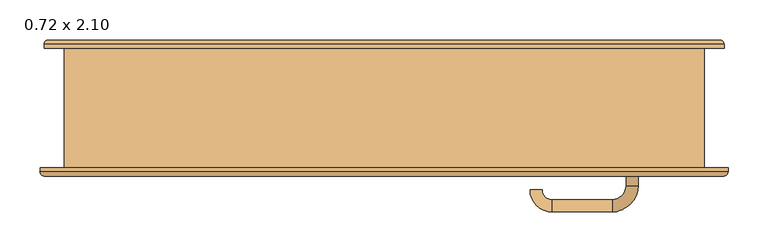
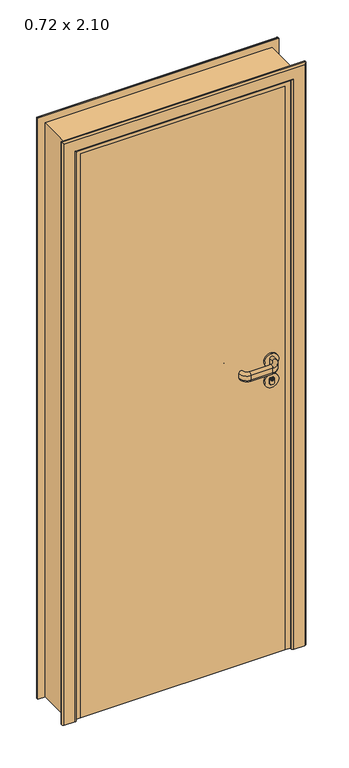
"""IFC4 building model written with IfcOpenShell, lengths in millimetres: door geometry, CC_PORTA ABRIR_1 FOLHA LISA : 0.72 x 2.10."""

from ifc_helpers import new_model, si_unit, point, frame, frame_2d, origin, origin_with_axes, place, context, project, spatial, polyline, circle_curve, ellipse_curve, trimmed, segment, composite_curve, outline, extrude, faceted_brep, source, transform, mapped, element, save
from ifc_brep_helpers import plane_surface, cylinder_surface, revolved_surface, advanced_brep


def door_0_72_x_2_10_8ac540cf(model_context):
    return source(origin(), model_context, "Body", "SolidModel", [
        advanced_brep(
        [(302.5, -40.0, 1091.5062746), (317.5, -40.0, 1091.5062746), (317.5, -40.0, 1108.3826844), (302.5, -40.0, 1108.3826844), (317.5, -18.0, 1091.5062746), (317.5, -18.0, 1108.3826844), (302.5, -18.0, 1108.3826844), (302.5, -18.0, 1091.5062746), (285.0, 14.5, 1108.3826844), (285.0, 14.5, 1091.5062746), (210.0, 14.5, 1091.5062746), (210.0, 14.5, 1108.3826844), (285.0, -0.5, 1091.5062746), (285.0, -0.5, 1108.3826844), (210.0, -0.5, 1108.3826844), (210.0, -0.5, 1091.5062746), (197.5, -13.0, 1091.5062746), (197.5, -13.0, 1108.3826844), (182.5, -13.0, 1108.3826844), (182.5, -13.0, 1091.5062746)],
        [
            (0, 1, circle_curve(frame((310.0, -40.0, 1091.5062746), z_axis=(0.0, -1.0, 0.0), x_axis=(0.0, 0.0, 1.0)), 7.5)),
            (1, 2),
            (2, 3, circle_curve(frame((310.0, -40.0, 1108.3826844), z_axis=(0.0, -1.0, 0.0), x_axis=(0.0, 0.0, 1.0)), 7.5)),
            (3, 0),
            (1, 4),
            (4, 5),
            (5, 2),
            (3, 6),
            (6, 7),
            (7, 0),
            (8, 9),
            (9, 10),
            (10, 11),
            (11, 8),
            (12, 13),
            (13, 14),
            (14, 15),
            (15, 12),
            (7, 4, circle_curve(frame((310.0, -18.0, 1091.5062746), z_axis=(0.0, -1.0, 0.0), x_axis=(0.0, 0.0, 1.0)), 7.5)),
            (5, 6, circle_curve(frame((310.0, -18.0, 1108.3826844), z_axis=(0.0, -1.0, 0.0), x_axis=(0.0, 0.0, 1.0)), 7.5)),
            (9, 12, circle_curve(frame((285.0, 7.0, 1091.5062746), z_axis=(-1.0, 0.0, 0.0), x_axis=(0.0, 0.0, 1.0)), 7.5)),
            (15, 10, circle_curve(frame((210.0, 7.0, 1091.5062746), z_axis=(1.0, 0.0, 0.0), x_axis=(0.0, 0.0, 1.0)), 7.5)),
            (13, 8, circle_curve(frame((285.0, 7.0, 1108.3826844), z_axis=(-1.0, 0.0, 0.0), x_axis=(0.0, 0.0, 1.0)), 7.5)),
            (11, 14, circle_curve(frame((210.0, 7.0, 1108.3826844), z_axis=(1.0, 0.0, 0.0), x_axis=(0.0, 0.0, 1.0)), 7.5)),
            (9, 4, circle_curve(frame((285.0, -18.0, 1091.5062746), z_axis=(0.0, 0.0, -1.0), x_axis=(1.0, 0.0, 0.0)), 32.5)),
            (7, 12, circle_curve(frame((285.0, -18.0, 1091.5062746), z_axis=(0.0, 0.0, 1.0), x_axis=(1.0, 0.0, 0.0)), 17.5)),
            (8, 5, circle_curve(frame((285.0, -18.0, 1108.3826844), z_axis=(0.0, 0.0, -1.0), x_axis=(1.0, 0.0, 0.0)), 32.5)),
            (13, 6, circle_curve(frame((285.0, -18.0, 1108.3826844), z_axis=(0.0, 0.0, -1.0), x_axis=(1.0, 0.0, 0.0)), 17.5)),
            (16, 17),
            (17, 18, circle_curve(frame((190.0, -13.0, 1108.3826844), z_axis=(0.0, -1.0, 0.0), x_axis=(0.0, 0.0, 1.0)), 7.5)),
            (18, 19),
            (19, 16, circle_curve(frame((190.0, -13.0, 1091.5062746), z_axis=(0.0, -1.0, 0.0), x_axis=(0.0, 0.0, 1.0)), 7.5)),
            (19, 10, circle_curve(frame((210.0, -13.0, 1091.5062746), z_axis=(0.0, 0.0, -1.0), x_axis=(0.0, 1.0, 0.0)), 27.5)),
            (15, 16, circle_curve(frame((210.0, -13.0, 1091.5062746), z_axis=(0.0, 0.0, 1.0), x_axis=(0.0, 1.0, 0.0)), 12.5)),
            (18, 11, circle_curve(frame((210.0, -13.0, 1108.3826844), z_axis=(0.0, 0.0, -1.0), x_axis=(0.0, 1.0, 0.0)), 27.5)),
            (17, 14, circle_curve(frame((210.0, -13.0, 1108.3826844), z_axis=(0.0, 0.0, -1.0), x_axis=(0.0, 1.0, 0.0)), 12.5)),
        ],
        [
            plane_surface(frame((310.0, -40.0, 1099.9444795), z_axis=(0.0, -1.0, 0.0), x_axis=(0.0, 0.0, 1.0))),
            plane_surface(frame((317.5, -40.0, 1091.5062746), z_axis=(1.0, 0.0, 0.0), x_axis=(0.0, 1.0, 0.0))),
            plane_surface(frame((302.5, -40.0, 1108.3826844), z_axis=(-1.0, 0.0, 0.0), x_axis=(0.0, 1.0, 0.0))),
            plane_surface(frame((285.0, 14.5, 1091.5062746), z_axis=(0.0, 1.0, 0.0), x_axis=(-1.0, 0.0, 0.0))),
            plane_surface(frame((285.0, -0.5, 1108.3826844), z_axis=(0.0, -1.0, 0.0), x_axis=(-1.0, 0.0, 0.0))),
            cylinder_surface(frame((310.0, -40.0, 1091.5062746), z_axis=(0.0, -1.0, 0.0), x_axis=(0.0, 0.0, 1.0)), 7.5),
            cylinder_surface(frame((310.0, -40.0, 1108.3826844), z_axis=(0.0, -1.0, 0.0), x_axis=(0.0, 0.0, 1.0)), 7.5),
            cylinder_surface(frame((285.0, 7.0, 1091.5062746), z_axis=(1.0, 0.0, 0.0), x_axis=(0.0, 0.0, 1.0)), 7.5),
            cylinder_surface(frame((285.0, 7.0, 1108.3826844), z_axis=(1.0, 0.0, 0.0), x_axis=(0.0, 0.0, 1.0)), 7.5),
            revolved_surface(trimmed(ellipse_curve(frame((310.0, -18.0, 1091.5062746), z_axis=(0.0, -1.0, 0.0), x_axis=(0.0, 0.0, 1.0)), 7.5, 7.5), [point((302.5, -18.0, 1091.5062746))], [point((317.5, -18.0, 1091.5062746))], True, "CARTESIAN"), (285.0, -18.0, 1099.9444795), (0.0, 0.0, 1.0)),
            cylinder_surface(frame((285.0, -18.0, 1099.9444795), z_axis=(0.0, 0.0, 1.0), x_axis=(1.0, 0.0, 0.0)), 32.5),
            revolved_surface(trimmed(ellipse_curve(frame((310.0, -18.0, 1108.3826844), z_axis=(0.0, -1.0, 0.0), x_axis=(0.0, 0.0, 1.0)), 7.5, 7.5), [point((317.5, -18.0, 1108.3826844))], [point((302.5, -18.0, 1108.3826844))], True, "CARTESIAN"), (285.0, -18.0, 1099.9444795), (0.0, 0.0, 1.0)),
            revolved_surface(polyline([(302.5, -18.0, 1108.3826844), (302.5, -18.0, 1091.5062746)]), (285.0, -18.0, 1099.9444795), (0.0, 0.0, 1.0)),
            plane_surface(frame((190.0, -13.0, 1099.9444795), z_axis=(0.0, -1.0, 0.0), x_axis=(0.0, 0.0, 1.0))),
            revolved_surface(trimmed(ellipse_curve(frame((210.0, 7.0, 1091.5062746), z_axis=(1.0, 0.0, 0.0), x_axis=(0.0, 0.0, 1.0)), 7.5, 7.5), [point((210.0, -0.5, 1091.5062746))], [point((210.0, 14.5, 1091.5062746))], True, "CARTESIAN"), (210.0, -13.0, 1099.9444795), (0.0, 0.0, 1.0)),
            cylinder_surface(frame((210.0, -13.0, 1099.9444795), z_axis=(0.0, 0.0, 1.0), x_axis=(0.0, 1.0, 0.0)), 27.5),
            revolved_surface(trimmed(ellipse_curve(frame((210.0, 7.0, 1108.3826844), z_axis=(1.0, 0.0, 0.0), x_axis=(0.0, 0.0, 1.0)), 7.5, 7.5), [point((210.0, 14.5, 1108.3826844))], [point((210.0, -0.5, 1108.3826844))], True, "CARTESIAN"), (210.0, -13.0, 1099.9444795), (0.0, 0.0, 1.0)),
            revolved_surface(polyline([(210.0, -0.5, 1108.3826844), (210.0, -0.5, 1091.5062746)]), (210.0, -13.0, 1099.9444795), (0.0, 0.0, 1.0)),
        ],
        [
            (0, [[1, 2, 3, 4]]),
            (1, [[-2, 5, 6, 7]]),
            (2, [[-4, 8, 9, 10]]),
            (3, [[11, 12, 13, 14]]),
            (4, [[15, 16, 17, 18]]),
            (5, [[-1, -10, 19, -5]]),
            (6, [[-3, -7, 20, -8]]),
            (7, [[21, -18, 22, -12]]),
            (8, [[23, -14, 24, -16]]),
            (9, [[25, -19, 26, -21]]),
            (10, [[27, -6, -25, -11]]),
            (11, [[28, -20, -27, -23]]),
            (12, [[-26, -9, -28, -15]]),
            (13, [[29, 30, 31, 32]]),
            (14, [[33, -22, 34, -32]]),
            (15, [[35, -13, -33, -31]]),
            (16, [[36, -24, -35, -30]]),
            (17, [[-34, -17, -36, -29]]),
        ],
    ),
        extrude(outline(polyline([(311.0, -40.0), (309.0, -40.0), (309.0, -30.9), (311.0, -30.9), (311.0, -40.0)])), frame((0.0, 0.0, 1027.9555433), z_axis=(0.0, 0.0, 1.0), x_axis=(1.0, 0.0, 0.0)), (0.0, 0.0, 1.0), 7.8071257),
        extrude(outline(composite_curve([segment(trimmed(circle_curve(frame_2d((1031.5611613, 310.0)), 5.0), [point((1036.5611613, 310.0))], [point((1026.5611613, 310.0))], False, "CARTESIAN"), True, "CONTINUOUS"), segment(trimmed(circle_curve(frame_2d((1031.5611613, 310.0)), 5.0), [point((1026.5611613, 310.0))], [point((1036.5611613, 310.0))], False, "CARTESIAN"), True, "CONTINUOUS")], self_intersect=False), holes=[polyline([(1035.7626689, 311.0), (1027.9555433, 311.0), (1027.9555433, 309.0), (1035.7626689, 309.0), (1035.7626689, 311.0)])]), frame((0.0, -40.0, 0.0), z_axis=(0.0, 1.0, 0.0), x_axis=(0.0, 0.0, 1.0)), (0.0, 0.0, 1.0), 10.0),
        extrude(outline(composite_curve([segment(polyline([(1033.4817325, 302.5), (1016.4817325, 302.5)]), True, "CONTINUOUS"), segment(trimmed(circle_curve(frame_2d((1016.4817325, 306.5)), 4.0), [point((1016.4817325, 302.5))], [point((1012.4817325, 306.5))], False, "CARTESIAN"), True, "CONTINUOUS"), segment(polyline([(1012.4817325, 306.5), (1012.4817325, 313.5)]), True, "CONTINUOUS"), segment(trimmed(circle_curve(frame_2d((1016.4817325, 313.5)), 4.0), [point((1012.4817325, 313.5))], [point((1016.4817325, 317.5))], False, "CARTESIAN"), True, "CONTINUOUS"), segment(polyline([(1016.4817325, 317.5), (1033.4817325, 317.5)]), True, "CONTINUOUS"), segment(trimmed(circle_curve(frame_2d((1033.4817325, 313.5)), 4.0), [point((1033.4817325, 317.5))], [point((1037.4817325, 313.5))], False, "CARTESIAN"), True, "CONTINUOUS"), segment(polyline([(1037.4817325, 313.5), (1037.4817325, 306.5)]), True, "CONTINUOUS"), segment(trimmed(circle_curve(frame_2d((1033.4817325, 306.5)), 4.0), [point((1037.4817325, 306.5))], [point((1033.4817325, 302.5))], False, "CARTESIAN"), True, "CONTINUOUS")], self_intersect=False)), frame((0.0, -40.0, 0.0), z_axis=(0.0, 1.0, 0.0), x_axis=(0.0, 0.0, 1.0)), (0.0, 0.0, 1.0), 9.0),
        extrude(outline(composite_curve([segment(trimmed(circle_curve(frame_2d((1099.9444795, 310.0)), 25.0), [point((1124.9444795, 310.0))], [point((1074.9444795, 310.0))], False, "CARTESIAN"), True, "CONTINUOUS"), segment(trimmed(circle_curve(frame_2d((1099.9444795, 310.0)), 25.0), [point((1074.9444795, 310.0))], [point((1124.9444795, 310.0))], False, "CARTESIAN"), True, "CONTINUOUS")], self_intersect=False)), frame((0.0, -40.0, 0.0), z_axis=(0.0, 1.0, 0.0), x_axis=(0.0, 0.0, 1.0)), (0.0, 0.0, 1.0), 6.0),
        extrude(outline(composite_curve([segment(trimmed(circle_curve(frame_2d((1024.9444795, 310.0)), 25.0), [point((1049.9444795, 310.0))], [point((999.9444795, 310.0))], False, "CARTESIAN"), True, "CONTINUOUS"), segment(trimmed(circle_curve(frame_2d((1024.9444795, 310.0)), 25.0), [point((999.9444795, 310.0))], [point((1049.9444795, 310.0))], False, "CARTESIAN"), True, "CONTINUOUS")], self_intersect=False), holes=[composite_curve([segment(trimmed(circle_curve(frame_2d((1033.4817325, 313.5)), 4.0), [point((1037.4817325, 313.5))], [point((1033.4817325, 317.5))], True, "CARTESIAN"), True, "CONTINUOUS"), segment(polyline([(1033.4817325, 317.5), (1016.4817325, 317.5)]), True, "CONTINUOUS"), segment(trimmed(circle_curve(frame_2d((1016.4817325, 313.5)), 4.0), [point((1016.4817325, 317.5))], [point((1012.4817325, 313.5))], True, "CARTESIAN"), True, "CONTINUOUS"), segment(polyline([(1012.4817325, 313.5), (1012.4817325, 306.5)]), True, "CONTINUOUS"), segment(trimmed(circle_curve(frame_2d((1016.4817325, 306.5)), 4.0), [point((1012.4817325, 306.5))], [point((1016.4817325, 302.5))], True, "CARTESIAN"), True, "CONTINUOUS"), segment(polyline([(1016.4817325, 302.5), (1033.4817325, 302.5)]), True, "CONTINUOUS"), segment(trimmed(circle_curve(frame_2d((1033.4817325, 306.5)), 4.0), [point((1033.4817325, 302.5))], [point((1037.4817325, 306.5))], True, "CARTESIAN"), True, "CONTINUOUS"), segment(polyline([(1037.4817325, 306.5), (1037.4817325, 313.5)]), True, "CONTINUOUS")], self_intersect=False)]), frame((0.0, -40.0, 0.0), z_axis=(0.0, 1.0, 0.0), x_axis=(0.0, 0.0, 1.0)), (0.0, 0.0, 1.0), 6.0),
        extrude(outline(polyline([(311.0, -84.1), (309.0, -84.1), (309.0, -75.0), (311.0, -75.0), (311.0, -84.1)])), frame((0.0, 0.0, 1027.9555433), z_axis=(0.0, 0.0, 1.0), x_axis=(1.0, 0.0, 0.0)), (0.0, 0.0, 1.0), 7.8071257),
        advanced_brep(
        [(310.0, -85.0, 1036.5611613), (310.0, -85.0, 1026.5611613), (311.0, -85.0, 1035.7626689), (311.0, -85.0, 1027.9555433), (309.0, -85.0, 1027.9555433), (309.0, -85.0, 1035.7626689), (310.0, -75.0, 1049.9444795), (310.0, -75.0, 999.9444795), (310.0, -84.0, 1036.5611613), (310.0, -84.0, 1026.5611613), (311.0, -84.0, 1035.7626689), (311.0, -84.0, 1027.9555433), (309.0, -84.0, 1027.9555433), (309.0, -84.0, 1035.7626689), (302.5, -84.0, 1033.4817325), (302.5, -84.0, 1016.4817325), (306.5, -84.0, 1012.4817325), (313.5, -84.0, 1012.4817325), (317.5, -84.0, 1016.4817325), (317.5, -84.0, 1033.4817325), (313.5, -84.0, 1037.4817325), (306.5, -84.0, 1037.4817325), (302.5, -81.0, 1033.4817325), (302.5, -81.0, 1016.4817325), (306.5, -81.0, 1012.4817325), (313.5, -81.0, 1012.4817325), (317.5, -81.0, 1016.4817325), (317.5, -81.0, 1033.4817325), (313.5, -81.0, 1037.4817325), (306.5, -81.0, 1037.4817325), (310.0, -81.0, 1049.9444795), (310.0, -81.0, 999.9444795)],
        [
            (0, 1, circle_curve(frame((310.0, -85.0, 1031.5611613), z_axis=(0.0, -1.0, 0.0), x_axis=(0.0, 0.0, -1.0)), 5.0)),
            (1, 0, circle_curve(frame((310.0, -85.0, 1031.5611613), z_axis=(0.0, -1.0, 0.0), x_axis=(0.0, 0.0, -1.0)), 5.0)),
            (2, 3),
            (3, 4),
            (4, 5),
            (5, 2),
            (6, 7, circle_curve(frame((310.0, -75.0, 1024.9444795), z_axis=(0.0, 1.0, 0.0), x_axis=(0.0, 0.0, -1.0)), 25.0)),
            (7, 6, circle_curve(frame((310.0, -75.0, 1024.9444795), z_axis=(0.0, 1.0, 0.0), x_axis=(0.0, 0.0, -1.0)), 25.0)),
            (0, 8),
            (8, 9, circle_curve(frame((310.0, -84.0, 1031.5611613), z_axis=(0.0, -1.0, 0.0), x_axis=(0.0, 0.0, -1.0)), 5.0)),
            (9, 1),
            (9, 8, circle_curve(frame((310.0, -84.0, 1031.5611613), z_axis=(0.0, -1.0, 0.0), x_axis=(0.0, 0.0, -1.0)), 5.0)),
            (2, 10),
            (10, 11),
            (11, 3),
            (11, 12),
            (12, 4),
            (12, 13),
            (13, 5),
            (13, 10),
            (14, 15),
            (15, 16, circle_curve(frame((306.5, -84.0, 1016.4817325), z_axis=(0.0, -1.0, 0.0), x_axis=(0.0, 0.0, -1.0)), 4.0)),
            (16, 17),
            (17, 18, circle_curve(frame((313.5, -84.0, 1016.4817325), z_axis=(0.0, -1.0, 0.0), x_axis=(0.0, 0.0, -1.0)), 4.0)),
            (18, 19),
            (19, 20, circle_curve(frame((313.5, -84.0, 1033.4817325), z_axis=(0.0, -1.0, 0.0), x_axis=(0.0, 0.0, -1.0)), 4.0)),
            (20, 21),
            (21, 14, circle_curve(frame((306.5, -84.0, 1033.4817325), z_axis=(0.0, -1.0, 0.0), x_axis=(0.0, 0.0, -1.0)), 4.0)),
            (14, 22),
            (22, 23),
            (23, 15),
            (23, 24, circle_curve(frame((306.5, -81.0, 1016.4817325), z_axis=(0.0, -1.0, 0.0), x_axis=(0.0, 0.0, -1.0)), 4.0)),
            (24, 16),
            (24, 25),
            (25, 17),
            (25, 26, circle_curve(frame((313.5, -81.0, 1016.4817325), z_axis=(0.0, -1.0, 0.0), x_axis=(0.0, 0.0, -1.0)), 4.0)),
            (26, 18),
            (26, 27),
            (27, 19),
            (27, 28, circle_curve(frame((313.5, -81.0, 1033.4817325), z_axis=(0.0, -1.0, 0.0), x_axis=(0.0, 0.0, -1.0)), 4.0)),
            (28, 20),
            (28, 29),
            (29, 21),
            (29, 22, circle_curve(frame((306.5, -81.0, 1033.4817325), z_axis=(0.0, -1.0, 0.0), x_axis=(0.0, 0.0, -1.0)), 4.0)),
            (30, 31, circle_curve(frame((310.0, -81.0, 1024.9444795), z_axis=(0.0, -1.0, 0.0), x_axis=(0.0, 0.0, -1.0)), 25.0)),
            (31, 30, circle_curve(frame((310.0, -81.0, 1024.9444795), z_axis=(0.0, -1.0, 0.0), x_axis=(0.0, 0.0, -1.0)), 25.0)),
            (30, 6),
            (7, 31),
        ],
        [
            plane_surface(frame((310.0, -85.0, 1026.5611613), z_axis=(0.0, -1.0, 0.0), x_axis=(1.0, 0.0, 0.0))),
            plane_surface(frame((310.0, -75.0, 1026.5611613), z_axis=(0.0, 1.0, 0.0), x_axis=(-1.0, 0.0, 0.0))),
            cylinder_surface(frame((310.0, -75.0, 1031.5611613), z_axis=(0.0, -1.0, 0.0), x_axis=(0.0, 0.0, -1.0)), 5.0),
            plane_surface(frame((311.0, -85.0, 1035.7626689), z_axis=(-1.0, 0.0, 0.0), x_axis=(0.0, 1.0, 0.0))),
            plane_surface(frame((311.0, -85.0, 1027.9555433), z_axis=(0.0, 0.0, 1.0), x_axis=(0.0, 1.0, 0.0))),
            plane_surface(frame((309.0, -85.0, 1027.9555433), z_axis=(1.0, 0.0, 0.0), x_axis=(0.0, 1.0, 0.0))),
            plane_surface(frame((309.0, -85.0, 1035.7626689), z_axis=(0.0, 0.0, -1.0), x_axis=(0.0, 1.0, 0.0))),
            plane_surface(frame((302.5, -84.0, 1016.4817325), z_axis=(0.0, -1.0, 0.0), x_axis=(0.0, 0.0, -1.0))),
            plane_surface(frame((302.5, -84.0, 1033.4817325), z_axis=(-1.0, 0.0, 0.0), x_axis=(0.0, 1.0, 0.0))),
            cylinder_surface(frame((306.5, -75.0, 1016.4817325), z_axis=(0.0, -1.0, 0.0), x_axis=(0.0, 0.0, -1.0)), 4.0),
            plane_surface(frame((306.5, -84.0, 1012.4817325), z_axis=(0.0, 0.0, -1.0), x_axis=(0.0, 1.0, 0.0))),
            cylinder_surface(frame((313.5, -75.0, 1016.4817325), z_axis=(0.0, -1.0, 0.0), x_axis=(0.0, 0.0, -1.0)), 4.0),
            plane_surface(frame((317.5, -84.0, 1016.4817325), z_axis=(1.0, 0.0, 0.0), x_axis=(0.0, 1.0, 0.0))),
            cylinder_surface(frame((313.5, -75.0, 1033.4817325), z_axis=(0.0, -1.0, 0.0), x_axis=(0.0, 0.0, -1.0)), 4.0),
            plane_surface(frame((313.5, -84.0, 1037.4817325), z_axis=(0.0, 0.0, 1.0), x_axis=(0.0, 1.0, 0.0))),
            cylinder_surface(frame((306.5, -75.0, 1033.4817325), z_axis=(0.0, -1.0, 0.0), x_axis=(0.0, 0.0, -1.0)), 4.0),
            plane_surface(frame((310.0, -81.0, 1074.9444795), z_axis=(0.0, -1.0, 0.0), x_axis=(1.0, 0.0, 0.0))),
            cylinder_surface(frame((310.0, -75.0, 1024.9444795), z_axis=(0.0, -1.0, 0.0), x_axis=(0.0, 0.0, -1.0)), 25.0),
        ],
        [
            (0, [[1, 2], [3, 4, 5, 6]]),
            (1, [[7, 8]]),
            (2, [[-1, 9, 10, 11]]),
            (2, [[-2, -11, 12, -9]]),
            (3, [[-3, 13, 14, 15]]),
            (4, [[-4, -15, 16, 17]]),
            (5, [[-5, -17, 18, 19]]),
            (6, [[-6, -19, 20, -13]]),
            (7, [[-14, -20, -18, -16]]),
            (7, [[21, 22, 23, 24, 25, 26, 27, 28], [-10, -12]]),
            (8, [[-21, 29, 30, 31]]),
            (9, [[-22, -31, 32, 33]]),
            (10, [[-23, -33, 34, 35]]),
            (11, [[-24, -35, 36, 37]]),
            (12, [[-25, -37, 38, 39]]),
            (13, [[-26, -39, 40, 41]]),
            (14, [[-27, -41, 42, 43]]),
            (15, [[-28, -43, 44, -29]]),
            (16, [[45, 46], [-30, -44, -42, -40, -38, -36, -34, -32]]),
            (17, [[-45, 47, -8, 48]]),
            (17, [[-46, -48, -7, -47]]),
        ],
    ),
        advanced_brep(
        [(310.0, -75.0, 1124.9444795), (310.0, -75.0, 1074.9444795), (310.0, -81.0, 1124.9444795), (310.0, -81.0, 1074.9444795)],
        [
            (0, 1, circle_curve(frame((310.0, -75.0, 1099.9444795), z_axis=(0.0, 1.0, 0.0), x_axis=(0.0, 0.0, -1.0)), 25.0)),
            (1, 0, circle_curve(frame((310.0, -75.0, 1099.9444795), z_axis=(0.0, 1.0, 0.0), x_axis=(0.0, 0.0, -1.0)), 25.0)),
            (2, 3, circle_curve(frame((310.0, -81.0, 1099.9444795), z_axis=(0.0, -1.0, 0.0), x_axis=(0.0, 0.0, -1.0)), 25.0)),
            (3, 2, circle_curve(frame((310.0, -81.0, 1099.9444795), z_axis=(0.0, -1.0, 0.0), x_axis=(0.0, 0.0, -1.0)), 25.0)),
            (2, 0),
            (1, 3),
        ],
        [
            plane_surface(frame((310.0, -75.0, 1026.5611613), z_axis=(0.0, 1.0, 0.0), x_axis=(-1.0, 0.0, 0.0))),
            plane_surface(frame((310.0, -81.0, 1074.9444795), z_axis=(0.0, -1.0, 0.0), x_axis=(1.0, 0.0, 0.0))),
            cylinder_surface(frame((310.0, -75.0, 1099.9444795), z_axis=(0.0, -1.0, 0.0), x_axis=(0.0, 0.0, -1.0)), 25.0),
        ],
        [
            (0, [[1, 2]]),
            (1, [[3, 4]]),
            (2, [[-3, 5, -2, 6]]),
            (2, [[-4, -6, -1, -5]]),
        ],
    ),
        advanced_brep(
        [(302.5, -75.0, 1108.4382049), (317.5, -75.0, 1108.4382049), (317.5, -75.0, 1091.5617951), (302.5, -75.0, 1091.5617951), (317.5, -97.0, 1108.4382049), (317.5, -97.0, 1091.5617951), (302.5, -97.0, 1091.5617951), (302.5, -97.0, 1108.4382049), (285.0, -129.5, 1091.5617951), (285.0, -129.5, 1108.4382049), (210.0, -129.5, 1108.4382049), (210.0, -129.5, 1091.5617951), (285.0, -114.5, 1108.4382049), (285.0, -114.5, 1091.5617951), (210.0, -114.5, 1091.5617951), (210.0, -114.5, 1108.4382049), (197.5, -102.0, 1108.4382049), (197.5, -102.0, 1091.5617951), (182.5, -102.0, 1091.5617951), (182.5, -102.0, 1108.4382049)],
        [
            (0, 1, circle_curve(frame((310.0, -75.0, 1108.4382049), z_axis=(0.0, 1.0, 0.0), x_axis=(-1.0, 0.0, 0.0)), 7.5)),
            (1, 2),
            (2, 3, circle_curve(frame((310.0, -75.0, 1091.5617951), z_axis=(0.0, 1.0, 0.0), x_axis=(-1.0, 0.0, 0.0)), 7.5)),
            (3, 0),
            (1, 4),
            (4, 5),
            (5, 2),
            (3, 6),
            (6, 7),
            (7, 0),
            (8, 9),
            (9, 10),
            (10, 11),
            (11, 8),
            (12, 13),
            (13, 14),
            (14, 15),
            (15, 12),
            (7, 4, circle_curve(frame((310.0, -97.0, 1108.4382049), z_axis=(0.0, 1.0, 0.0), x_axis=(-1.0, 0.0, 0.0)), 7.5)),
            (5, 6, circle_curve(frame((310.0, -97.0, 1091.5617951), z_axis=(0.0, 1.0, 0.0), x_axis=(-1.0, 0.0, 0.0)), 7.5)),
            (9, 12, circle_curve(frame((285.0, -122.0, 1108.4382049), z_axis=(-1.0, 0.0, 0.0), x_axis=(0.0, 1.0, 0.0)), 7.5)),
            (15, 10, circle_curve(frame((210.0, -122.0, 1108.4382049), z_axis=(1.0, 0.0, 0.0), x_axis=(0.0, 1.0, 0.0)), 7.5)),
            (13, 8, circle_curve(frame((285.0, -122.0, 1091.5617951), z_axis=(-1.0, 0.0, 0.0), x_axis=(0.0, 1.0, 0.0)), 7.5)),
            (11, 14, circle_curve(frame((210.0, -122.0, 1091.5617951), z_axis=(1.0, 0.0, 0.0), x_axis=(0.0, 1.0, 0.0)), 7.5)),
            (9, 4, circle_curve(frame((285.0, -97.0, 1108.4382049), z_axis=(0.0, 0.0, 1.0), x_axis=(1.0, 0.0, 0.0)), 32.5)),
            (7, 12, circle_curve(frame((285.0, -97.0, 1108.4382049), z_axis=(0.0, 0.0, -1.0), x_axis=(1.0, 0.0, 0.0)), 17.5)),
            (8, 5, circle_curve(frame((285.0, -97.0, 1091.5617951), z_axis=(0.0, 0.0, 1.0), x_axis=(1.0, 0.0, 0.0)), 32.5)),
            (13, 6, circle_curve(frame((285.0, -97.0, 1091.5617951), z_axis=(0.0, 0.0, 1.0), x_axis=(1.0, 0.0, 0.0)), 17.5)),
            (16, 17),
            (17, 18, circle_curve(frame((190.0, -102.0, 1091.5617951), z_axis=(0.0, 1.0, 0.0), x_axis=(1.0, 0.0, 0.0)), 7.5)),
            (18, 19),
            (19, 16, circle_curve(frame((190.0, -102.0, 1108.4382049), z_axis=(0.0, 1.0, 0.0), x_axis=(1.0, 0.0, 0.0)), 7.5)),
            (19, 10, circle_curve(frame((210.0, -102.0, 1108.4382049), z_axis=(0.0, 0.0, 1.0), x_axis=(0.0, -1.0, 0.0)), 27.5)),
            (15, 16, circle_curve(frame((210.0, -102.0, 1108.4382049), z_axis=(0.0, 0.0, -1.0), x_axis=(0.0, -1.0, 0.0)), 12.5)),
            (18, 11, circle_curve(frame((210.0, -102.0, 1091.5617951), z_axis=(0.0, 0.0, 1.0), x_axis=(0.0, -1.0, 0.0)), 27.5)),
            (17, 14, circle_curve(frame((210.0, -102.0, 1091.5617951), z_axis=(0.0, 0.0, 1.0), x_axis=(0.0, -1.0, 0.0)), 12.5)),
        ],
        [
            plane_surface(frame((310.0, -75.0, 1100.0), z_axis=(0.0, 1.0, 0.0), x_axis=(0.0, 0.0, -1.0))),
            plane_surface(frame((317.5, -75.0, 1108.4382049), z_axis=(1.0, 0.0, 0.0), x_axis=(0.0, -1.0, 0.0))),
            plane_surface(frame((302.5, -75.0, 1091.5617951), z_axis=(-1.0, 0.0, 0.0), x_axis=(0.0, -1.0, 0.0))),
            plane_surface(frame((285.0, -129.5, 1108.4382049), z_axis=(0.0, -1.0, 0.0), x_axis=(-1.0, 0.0, 0.0))),
            plane_surface(frame((285.0, -114.5, 1091.5617951), z_axis=(0.0, 1.0, 0.0), x_axis=(-1.0, 0.0, 0.0))),
            cylinder_surface(frame((310.0, -75.0, 1108.4382049), z_axis=(0.0, 1.0, 0.0), x_axis=(-1.0, 0.0, 0.0)), 7.5),
            cylinder_surface(frame((310.0, -75.0, 1091.5617951), z_axis=(0.0, 1.0, 0.0), x_axis=(-1.0, 0.0, 0.0)), 7.5),
            cylinder_surface(frame((285.0, -122.0, 1108.4382049), z_axis=(1.0, 0.0, 0.0), x_axis=(0.0, 1.0, 0.0)), 7.5),
            cylinder_surface(frame((285.0, -122.0, 1091.5617951), z_axis=(1.0, 0.0, 0.0), x_axis=(0.0, 1.0, 0.0)), 7.5),
            revolved_surface(trimmed(ellipse_curve(frame((310.0, -97.0, 1108.4382049), z_axis=(0.0, 1.0, 0.0), x_axis=(-1.0, 0.0, 0.0)), 7.5, 7.5), [point((302.5, -97.0, 1108.4382049))], [point((317.5, -97.0, 1108.4382049))], True, "CARTESIAN"), (285.0, -97.0, 1100.0), (0.0, 0.0, -1.0)),
            cylinder_surface(frame((285.0, -97.0, 1100.0), z_axis=(0.0, 0.0, -1.0), x_axis=(1.0, 0.0, 0.0)), 32.5),
            revolved_surface(trimmed(ellipse_curve(frame((310.0, -97.0, 1091.5617951), z_axis=(0.0, 1.0, 0.0), x_axis=(-1.0, 0.0, 0.0)), 7.5, 7.5), [point((317.5, -97.0, 1091.5617951))], [point((302.5, -97.0, 1091.5617951))], True, "CARTESIAN"), (285.0, -97.0, 1100.0), (0.0, 0.0, -1.0)),
            revolved_surface(polyline([(302.5, -97.0, 1091.5617951), (302.5, -97.0, 1108.4382049)]), (285.0, -97.0, 1100.0), (0.0, 0.0, -1.0)),
            plane_surface(frame((190.0, -102.0, 1100.0), z_axis=(0.0, 1.0, 0.0), x_axis=(0.0, 0.0, -1.0))),
            revolved_surface(trimmed(ellipse_curve(frame((210.0, -122.0, 1108.4382049), z_axis=(1.0, 0.0, 0.0), x_axis=(0.0, 1.0, 0.0)), 7.5, 7.5), [point((210.0, -114.5, 1108.4382049))], [point((210.0, -129.5, 1108.4382049))], True, "CARTESIAN"), (210.0, -102.0, 1100.0), (0.0, 0.0, -1.0)),
            cylinder_surface(frame((210.0, -102.0, 1100.0), z_axis=(0.0, 0.0, -1.0), x_axis=(0.0, -1.0, 0.0)), 27.5),
            revolved_surface(trimmed(ellipse_curve(frame((210.0, -122.0, 1091.5617951), z_axis=(1.0, 0.0, 0.0), x_axis=(0.0, 1.0, 0.0)), 7.5, 7.5), [point((210.0, -129.5, 1091.5617951))], [point((210.0, -114.5, 1091.5617951))], True, "CARTESIAN"), (210.0, -102.0, 1100.0), (0.0, 0.0, -1.0)),
            revolved_surface(polyline([(210.0, -114.5, 1091.5617951), (210.0, -114.5, 1108.4382049)]), (210.0, -102.0, 1100.0), (0.0, 0.0, -1.0)),
        ],
        [
            (0, [[1, 2, 3, 4]]),
            (1, [[-2, 5, 6, 7]]),
            (2, [[-4, 8, 9, 10]]),
            (3, [[11, 12, 13, 14]]),
            (4, [[15, 16, 17, 18]]),
            (5, [[-1, -10, 19, -5]]),
            (6, [[-3, -7, 20, -8]]),
            (7, [[21, -18, 22, -12]]),
            (8, [[23, -14, 24, -16]]),
            (9, [[25, -19, 26, -21]]),
            (10, [[27, -6, -25, -11]]),
            (11, [[28, -20, -27, -23]]),
            (12, [[-26, -9, -28, -15]]),
            (13, [[29, 30, 31, 32]]),
            (14, [[33, -22, 34, -32]]),
            (15, [[35, -13, -33, -31]]),
            (16, [[36, -24, -35, -30]]),
            (17, [[-34, -17, -36, -29]]),
        ],
    ),
        extrude(outline(polyline([(360.0, -75.0), (-360.0, -75.0), (-360.0, -40.0), (360.0, -40.0), (360.0, -75.0)])), origin_with_axes(), (0.0, 0.0, 1.0), 2100.0),
        advanced_brep(
        [(-380.5, 85.0, 0.0), (-375.0, 79.5, 0.0), (-375.0, 75.0, 0.0), (-425.0, 75.0, 0.0), (-425.0, 79.500573, 0.0), (-419.500573, 85.0, 0.0), (-380.5, 85.0, 2120.5), (-375.0, 79.5, 2115.0), (-375.0, 75.0, 2115.0), (375.0, 75.0, 2115.0), (375.0, 75.0, 0.0), (425.0, 75.0, 0.0), (425.0, 75.0, 2165.0), (-425.0, 75.0, 2165.0), (-425.0, 79.500573, 2165.0), (-419.500573, 85.0, 2159.500573), (419.500573, 85.0, 2159.500573), (419.500573, 85.0, 0.0), (380.5, 85.0, 0.0), (380.5, 85.0, 2120.5), (375.0, 79.5, 2115.0), (375.0, 79.5, 0.0), (425.0, 79.500573, 0.0), (425.0, 79.500573, 2165.0)],
        [
            (0, 1, circle_curve(frame((-380.5, 79.5, 0.0), z_axis=(0.0, 0.0, -1.0), x_axis=(0.0, 1.0, 0.0)), 5.5)),
            (1, 2),
            (2, 3),
            (3, 4),
            (4, 5, circle_curve(frame((-419.500573, 79.500573, 0.0), z_axis=(0.0, 0.0, -1.0), x_axis=(0.0, 1.0, 0.0)), 5.499427)),
            (5, 0),
            (0, 6),
            (6, 7, ellipse_curve(frame((-380.5, 79.5, 2120.5), z_axis=(-0.7071067811865475, 0.0, -0.7071067811865476), x_axis=(0.7071067811865476, 0.0, -0.7071067811865474)), 7.7781746, 5.5)),
            (7, 1),
            (7, 8),
            (8, 2),
            (8, 9),
            (9, 10),
            (10, 11),
            (11, 12),
            (12, 13),
            (13, 3),
            (13, 14),
            (14, 4),
            (14, 15, ellipse_curve(frame((-419.500573, 79.500573, 2159.500573), z_axis=(-0.7071067811865475, 0.0, -0.7071067811865476), x_axis=(0.7071067811865476, 0.0, -0.7071067811865474)), 7.7773642, 5.499427)),
            (15, 5),
            (15, 16),
            (16, 17),
            (17, 18),
            (18, 19),
            (19, 6),
            (9, 20),
            (20, 21),
            (21, 10),
            (17, 22, circle_curve(frame((419.500573, 79.500573, 0.0), z_axis=(0.0, 0.0, -1.0), x_axis=(0.0, 1.0, 0.0)), 5.499427)),
            (22, 11),
            (21, 18, circle_curve(frame((380.5, 79.5, 0.0), z_axis=(0.0, 0.0, -1.0), x_axis=(0.0, 1.0, 0.0)), 5.5)),
            (23, 12),
            (22, 23),
            (16, 23, ellipse_curve(frame((419.500573, 79.500573, 2159.500573), z_axis=(0.7071067811865475, 0.0, -0.7071067811865475), x_axis=(0.7071067811865474, 0.0, 0.7071067811865477)), 7.7773642, 5.499427)),
            (20, 19, ellipse_curve(frame((380.5, 79.5, 2120.5), z_axis=(0.7071067811865475, 0.0, -0.7071067811865475), x_axis=(0.7071067811865474, 0.0, 0.7071067811865477)), 7.7781746, 5.5)),
            (20, 7),
            (23, 14),
        ],
        [
            plane_surface(frame((-400.0, 75.0, 0.0), z_axis=(0.0, 0.0, -1.0), x_axis=(-1.0, 0.0, 0.0))),
            cylinder_surface(frame((-380.5, 79.5, 0.0), z_axis=(0.0, 0.0, -1.0), x_axis=(0.0, 1.0, 0.0)), 5.5),
            plane_surface(frame((-375.0, 79.5, 0.0), z_axis=(1.0, 0.0, 0.0), x_axis=(0.0, 0.0, 1.0))),
            plane_surface(frame((-375.0, 75.0, 0.0), z_axis=(0.0, -1.0, 0.0), x_axis=(0.0, 0.0, 1.0))),
            plane_surface(frame((-425.0, 75.0, 0.0), z_axis=(-1.0, 0.0, 0.0), x_axis=(0.0, 0.0, 1.0))),
            cylinder_surface(frame((-419.500573, 79.500573, 0.0), z_axis=(0.0, 0.0, -1.0), x_axis=(0.0, 1.0, 0.0)), 5.499427),
            plane_surface(frame((-419.500573, 85.0, 0.0), z_axis=(0.0, 1.0, 0.0), x_axis=(0.0, 0.0, 1.0))),
            plane_surface(frame((375.0, 79.5, 2115.0), z_axis=(-1.0, 0.0, 0.0), x_axis=(0.0, 0.0, -1.0))),
            plane_surface(frame((400.0, 75.0, 0.0), z_axis=(0.0, 0.0, -1.0), x_axis=(1.0, 0.0, 0.0))),
            plane_surface(frame((425.0, 75.0, 2165.0), z_axis=(1.0, 0.0, 0.0), x_axis=(0.0, 0.0, -1.0))),
            cylinder_surface(frame((419.500573, 79.500573, 2140.0), z_axis=(0.0, 0.0, 1.0), x_axis=(0.0, 1.0, 0.0)), 5.499427),
            cylinder_surface(frame((380.5, 79.5, 2140.0), z_axis=(0.0, 0.0, 1.0), x_axis=(0.0, 1.0, 0.0)), 5.5),
            cylinder_surface(frame((-400.0, 79.5, 2120.5), z_axis=(-1.0, 0.0, 0.0), x_axis=(0.0, 1.0, 0.0)), 5.5),
            plane_surface(frame((-375.0, 79.5, 2115.0), z_axis=(0.0, 0.0, -1.0), x_axis=(1.0, 0.0, 0.0))),
            plane_surface(frame((-425.0, 75.0, 2165.0), z_axis=(0.0, 0.0, 1.0), x_axis=(1.0, 0.0, 0.0))),
            cylinder_surface(frame((-400.0, 79.500573, 2159.500573), z_axis=(-1.0, 0.0, 0.0), x_axis=(0.0, 1.0, 0.0)), 5.499427),
        ],
        [
            (0, [[1, 2, 3, 4, 5, 6]]),
            (1, [[-1, 7, 8, 9]]),
            (2, [[-2, -9, 10, 11]]),
            (3, [[-3, -11, 12, 13, 14, 15, 16, 17]]),
            (4, [[-4, -17, 18, 19]]),
            (5, [[-5, -19, 20, 21]]),
            (6, [[-6, -21, 22, 23, 24, 25, 26, -7]]),
            (7, [[27, 28, 29, -13]]),
            (8, [[-24, 30, 31, -14, -29, 32]]),
            (9, [[33, -15, -31, 34]]),
            (10, [[35, -34, -30, -23]]),
            (11, [[36, -25, -32, -28]]),
            (12, [[-8, -26, -36, 37]]),
            (13, [[-10, -37, -27, -12]]),
            (14, [[-18, -16, -33, 38]]),
            (15, [[-20, -38, -35, -22]]),
        ],
    ),
        advanced_brep(
        [(-380.0, -75.0, 0.0), (-380.0, -79.5, 0.0), (-385.5, -85.0, 0.0), (-424.5, -85.0, 0.0), (-430.0, -79.5, 0.0), (-430.0, -75.0, 0.0), (-380.0, -75.0, 2120.0), (-380.0, -79.5, 2120.0), (-385.5, -85.0, 2125.5), (385.5, -85.0, 2125.5), (385.5, -85.0, 0.0), (424.5, -85.0, 0.0), (424.5, -85.0, 2164.5), (-424.5, -85.0, 2164.5), (-430.0, -79.5, 2170.0), (-430.0, -75.0, 2170.0), (430.0, -75.0, 2170.0), (430.0, -75.0, 0.0), (380.0, -75.0, 0.0), (380.0, -75.0, 2120.0), (380.0, -79.5, 2120.0), (380.0, -79.5, 0.0), (430.0, -79.5, 0.0), (430.0, -79.5, 2170.0)],
        [
            (0, 1),
            (1, 2, circle_curve(frame((-385.5, -79.5, 0.0), z_axis=(0.0, 0.0, -1.0), x_axis=(0.0, 1.0, 0.0)), 5.5)),
            (2, 3),
            (3, 4, circle_curve(frame((-424.5, -79.5, 0.0), z_axis=(0.0, 0.0, -1.0), x_axis=(0.0, 1.0, 0.0)), 5.5)),
            (4, 5),
            (5, 0),
            (0, 6),
            (6, 7),
            (7, 1),
            (7, 8, ellipse_curve(frame((-385.5, -79.5, 2125.5), z_axis=(-0.7071067811865475, 0.0, -0.7071067811865476), x_axis=(0.7071067811865476, 0.0, -0.7071067811865474)), 7.7781746, 5.5)),
            (8, 2),
            (8, 9),
            (9, 10),
            (10, 11),
            (11, 12),
            (12, 13),
            (13, 3),
            (13, 14, ellipse_curve(frame((-424.5, -79.5, 2164.5), z_axis=(-0.7071067811865475, 0.0, -0.7071067811865476), x_axis=(0.7071067811865476, 0.0, -0.7071067811865474)), 7.7781746, 5.5)),
            (14, 4),
            (14, 15),
            (15, 5),
            (15, 16),
            (16, 17),
            (17, 18),
            (18, 19),
            (19, 6),
            (9, 20, ellipse_curve(frame((385.5, -79.5, 2125.5), z_axis=(0.7071067811865475, 0.0, -0.7071067811865475), x_axis=(0.7071067811865474, 0.0, 0.7071067811865477)), 7.7781746, 5.5)),
            (20, 21),
            (21, 10, circle_curve(frame((385.5, -79.5, 0.0), z_axis=(0.0, 0.0, 1.0), x_axis=(0.0, 1.0, 0.0)), 5.5)),
            (17, 22),
            (22, 11, circle_curve(frame((424.5, -79.5, 0.0), z_axis=(0.0, 0.0, -1.0), x_axis=(0.0, 1.0, 0.0)), 5.5)),
            (21, 18),
            (23, 12, ellipse_curve(frame((424.5, -79.5, 2164.5), z_axis=(0.7071067811865475, 0.0, -0.7071067811865475), x_axis=(0.7071067811865474, 0.0, 0.7071067811865477)), 7.7781746, 5.5)),
            (22, 23),
            (16, 23),
            (20, 19),
            (20, 7),
            (23, 14),
        ],
        [
            plane_surface(frame((-400.0, -75.0, 0.0), z_axis=(0.0, 0.0, -1.0), x_axis=(-1.0, 0.0, 0.0))),
            plane_surface(frame((-380.0, -75.0, 0.0), z_axis=(1.0, 0.0, 0.0), x_axis=(0.0, 0.0, 1.0))),
            cylinder_surface(frame((-385.5, -79.5, 0.0), z_axis=(0.0, 0.0, -1.0), x_axis=(0.0, 1.0, 0.0)), 5.5),
            plane_surface(frame((-385.5, -85.0, 0.0), z_axis=(0.0, -1.0, 0.0), x_axis=(0.0, 0.0, 1.0))),
            cylinder_surface(frame((-424.5, -79.5, 0.0), z_axis=(0.0, 0.0, -1.0), x_axis=(0.0, 1.0, 0.0)), 5.5),
            plane_surface(frame((-430.0, -79.5, 0.0), z_axis=(-1.0, 0.0, 0.0), x_axis=(0.0, 0.0, 1.0))),
            plane_surface(frame((-430.0, -75.0, 0.0), z_axis=(0.0, 1.0, 0.0), x_axis=(0.0, 0.0, 1.0))),
            cylinder_surface(frame((385.5, -79.5, 2140.0), z_axis=(0.0, 0.0, 1.0), x_axis=(0.0, 1.0, 0.0)), 5.5),
            plane_surface(frame((400.0, -75.0, 0.0), z_axis=(0.0, 0.0, -1.0), x_axis=(1.0, 0.0, 0.0))),
            cylinder_surface(frame((424.5, -79.5, 2140.0), z_axis=(0.0, 0.0, 1.0), x_axis=(0.0, 1.0, 0.0)), 5.5),
            plane_surface(frame((430.0, -79.5, 2170.0), z_axis=(1.0, 0.0, 0.0), x_axis=(0.0, 0.0, -1.0))),
            plane_surface(frame((380.0, -75.0, 2120.0), z_axis=(-1.0, 0.0, 0.0), x_axis=(0.0, 0.0, -1.0))),
            plane_surface(frame((-380.0, -75.0, 2120.0), z_axis=(0.0, 0.0, -1.0), x_axis=(1.0, 0.0, 0.0))),
            cylinder_surface(frame((-400.0, -79.5, 2125.5), z_axis=(-1.0, 0.0, 0.0), x_axis=(0.0, 1.0, 0.0)), 5.5),
            cylinder_surface(frame((-400.0, -79.5, 2164.5), z_axis=(-1.0, 0.0, 0.0), x_axis=(0.0, 1.0, 0.0)), 5.5),
            plane_surface(frame((-430.0, -79.5, 2170.0), z_axis=(0.0, 0.0, 1.0), x_axis=(1.0, 0.0, 0.0))),
        ],
        [
            (0, [[1, 2, 3, 4, 5, 6]]),
            (1, [[-1, 7, 8, 9]]),
            (2, [[-2, -9, 10, 11]]),
            (3, [[-3, -11, 12, 13, 14, 15, 16, 17]]),
            (4, [[-4, -17, 18, 19]]),
            (5, [[-5, -19, 20, 21]]),
            (6, [[-6, -21, 22, 23, 24, 25, 26, -7]]),
            (7, [[27, 28, 29, -13]]),
            (8, [[-24, 30, 31, -14, -29, 32]]),
            (9, [[33, -15, -31, 34]]),
            (10, [[35, -34, -30, -23]]),
            (11, [[36, -25, -32, -28]]),
            (12, [[-8, -26, -36, 37]]),
            (13, [[-10, -37, -27, -12]]),
            (14, [[-18, -16, -33, 38]]),
            (15, [[-20, -38, -35, -22]]),
        ],
    ),
        faceted_brep([(-360.0, -40.0, 0.0), (-360.0, -75.0, 0.0), (-400.0, -75.0, 0.0), (-400.0, 75.0, 0.0), (-350.0, 75.0, 0.0), (-350.0, -40.0, 0.0), (-360.0, -40.0, 2100.0), (-360.0, -75.0, 2100.0), (360.0, -75.0, 2100.0), (360.0, -75.0, 0.0), (400.0, -75.0, 0.0), (400.0, -75.0, 2140.0), (-400.0, -75.0, 2140.0), (-400.0, 75.0, 2140.0), (400.0, 75.0, 2140.0), (400.0, 75.0, 0.0), (350.0, 75.0, 0.0), (350.0, 75.0, 2090.0), (-350.0, 75.0, 2090.0), (-350.0, -40.0, 2090.0), (350.0, -40.0, 2090.0), (350.0, -40.0, 0.0), (360.0, -40.0, 0.0), (360.0, -40.0, 2100.0)], [[[0, 1, 2, 3, 4, 5]], [[1, 0, 6, 7]], [[2, 1, 7, 8, 9, 10, 11, 12]], [[3, 2, 12, 13]], [[4, 3, 13, 14, 15, 16, 17, 18]], [[5, 4, 18, 19]], [[0, 5, 19, 20, 21, 22, 23, 6]], [[8, 23, 22, 9]], [[22, 21, 16, 15, 10, 9]], [[14, 11, 10, 15]], [[20, 17, 16, 21]], [[7, 6, 23, 8]], [[13, 12, 11, 14]], [[19, 18, 17, 20]]]),
    ])


if __name__ == "__main__":
    model = new_model("IFC4")
    model_context = context("Model", 3, world=origin())
    ifc_project = project(units=[si_unit("LENGTHUNIT", "METRE", prefix="MILLI")], contexts=[model_context])
    site = spatial("IfcSite", under=ifc_project)
    building = spatial("IfcBuilding", under=site)
    placement = place(None, origin())
    door_0_72_x_2_10_shape = door_0_72_x_2_10_8ac540cf(model_context)
    element("IfcDoor", 1, ObjectType="CC_PORTA ABRIR_1 FOLHA LISA : 0.72 x 2.10", at=placement, inside=building, context=model_context, shape_type="MappedRepresentation", body=[
        mapped(door_0_72_x_2_10_shape, transform((0.0, 0.0, 0.0), x_axis=(1.0, 0.0, 0.0), y_axis=(0.0, 1.0, 0.0), z_axis=(0.0, 0.0, 1.0))),
    ])
    save(model, "model.ifc")

# Revit data of these elements
# Type "CC_PORTA ABRIR_1 FOLHA LISA : 0.72 x 2.10"
#   Type Mark = "P5"
#   Site = "www.construir.arq.br"
#   Empresa = "Cursos Construir"
#   Description = "PORTA ABRIR 1 FOLHA LISA"
#   Criado Por = "Roberto Netto"
#   Analytic Construction = "<Nenhum>"
#   Atualizado por = "Rudemberg Eloi"
#   Rough Width = 0.80 m
#   Interna [instance default] = 0.00 m
#   Largura Guarnição Interna [instance default] = 0.05 m
#   Largura Guarnição Externa [instance default] = 0.05 m
#   Largura Folha [instance default] = 0.72 m
#   Externa [instance default] = 0.00 m
#   Extensão Lateral Esquerda [instance default] = 0.03 m
#   Extensão Lateral Direita [instance default] = 0.03 m
#   Extensão Frontal [instance default] = 0.03 m
#   Espessura Soleira [instance default] = 0.02 m
#   Espessura Guarnição Interna [instance default] = 0.01 m
#   Espessura Guarnição Externa [instance default] = 0.01 m
#   Espessura Folha [instance default] = 0.035 m
#   Espessura Batente [instance default] = 0.05 m
#   Eixo Rotação Folha [instance default] = 0.04 m
#   Deslocamento Maçaneta [instance default] = 0.05 m
#   Deslocamento Fechadura [instance default] = 0.05 m
#   Desloc (Interno) [instance default] = 0.02 m
#   Desloc (Externo) [instance default] = 0.025 m
#   Rough Height = 2.14 m
#   Altura Maçaneta [instance default] = 1.10 m
#   Altura Folha [instance default] = 2.10 m
#   Altura Fechadura [instance default] = 1.00 m
#   Height = 2.14 m
#   Width = 0.80 m
#   ----SOLEIRA---- [instance default] = 0.00 m
#   ----MAÇANETA/FECHADURA---- [instance default] = 0.00 m
#   ----GUARNIÇÃO---- [instance default] = 0.00 m
#   ----FOLHA---- [instance default] = 0.00 m
#   ----EXTENSÃO---- [instance default] = 0.00 m
#   ----BATENTE---- [instance default] = 0.00 m
#   Soleira Sem Extensão [instance default] = yes
#   Soleira Com Extensão [instance default] = no
#   Soleira [instance default] = yes
#   Maçaneta / Puxador [instance default] = yes
#   Guarnição Interna [instance default] = yes
#   Guarnição Externa [instance default] = yes
#   Fechadura Separada [instance default] = no
#   Bit [instance default] = no
#   Porcent. Exibição Batente Interno [instance default] = 50
#   Porcent. Exibição Batente Externo [instance default] = 50
#   Material Bit/Soleira = .GRANITO BRANCO ITAÚNAS
#   Material Espelho/Fixação = .AÇO INOXIDÁVEL ESCOVADO
#   Material Maçaneta/Puxador = .AÇO INOXIDÁVEL ESCOVADO
#   Material Guarnição Interna = .MADEIRA COM PINTURA ESMALTE BRANCO ACETINADO
#   Material Guarnição Externa = .MADEIRA COM PINTURA ESMALTE BRANCO ACETINADO
#   Material Folha = .MADEIRA COM PINTURA ESMALTE BRANCO ACETINADO
#   Material Fechadura = .AÇO INOXIDÁVEL ESCOVADO
#   Material Batente = .MADEIRA COM PINTURA ESMALTE BRANCO ACETINADO
#   Família Maçaneta [instance default] = element 1947931
#   Function = (empty or 0)
#   Wall Closure = (empty or 0)
# Element 1 (IfcDoor, "CC_PORTA ABRIR_1 FOLHA LISA : 0.72 x 2.10")
#   Materials on its faces: ".AÇO INOXIDÁVEL ESCOVADO", ".MADEIRA COM PINTURA ESMALTE BRANCO ACETINADO"
# Materials
#   ".GRANITO BRANCO ITAÚNAS": class ".CC_PEDRA REVEST.", colour RGB 202 195 174, transparency 0, Description = "Granito branco Itaúnas", Uso = "Pedra", Cost = 0
#   ".AÇO INOXIDÁVEL ESCOVADO": class "Metal", colour RGB 189 187 185, transparency 0, Description = "Stainless Steel 18/8, brushed finish", Cost = 0
#   ".MADEIRA COM PINTURA ESMALTE BRANCO ACETINADO": class ".CC_MADEIRAS", colour RGB 240 240 240, transparency 0, Description = "Madeira com pintura esmalte branco acetinado.", Cost = 0
